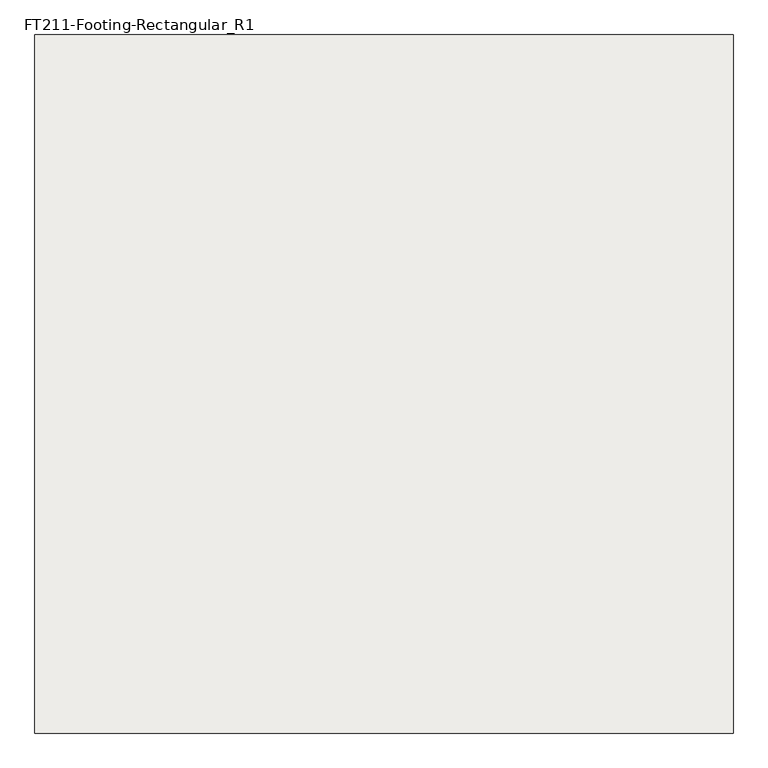
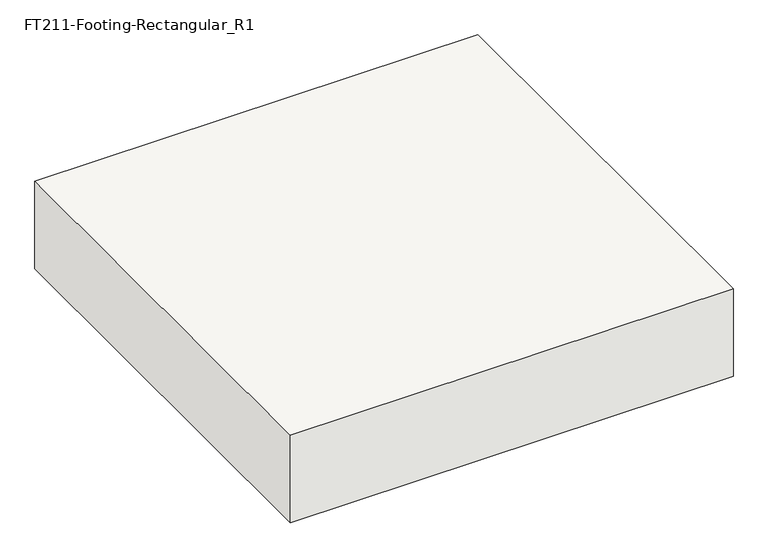
"""IFC4 building model written with IfcOpenShell, lengths in millimetres: slab geometry, FT211-Footing-Rectangular_R1 : H_SF_ACF_W2400xL2400xT500_Bitumen."""

import ifcopenshell
import ifcopenshell.guid

model = None  # the IFC model being written
_history = None  # IfcOwnerHistory: only IFC2X3 demands one
_inside = {}  # id of a spatial element -> (the spatial element, [elements in it])
_under = {}  # id of a project, library or spatial element -> (it, [spatial elements below it])
_declared = {}  # id of a project -> (the project, [libraries it declares])
_typed = {}  # id of a type object -> (the type object, [elements of that type])
_made_of = {}  # id of a material, layer set ... -> (it, [elements and type objects made of it])


def new_model(schema):
    """Start an empty IFC model of exactly this schema.

    Asked for "IFC4X3", IfcOpenShell would pick the latest addendum, in which some entities
    have other attributes; the version numbers below select the first issue.
    IFC2X3 requires an IfcOwnerHistory on every rooted entity: one is made here for all.
    """
    global model, _history
    if schema == "IFC4X3":
        model = ifcopenshell.file(schema_version=(4, 3, 0, 0))
    else:
        model = ifcopenshell.file(schema=schema)
    _inside.clear()
    _under.clear()
    _declared.clear()
    _typed.clear()
    _made_of.clear()
    _history = None
    if model.schema == "IFC2X3":
        org = make("IfcOrganization", Name="unknown")
        user = make(
            "IfcPersonAndOrganization",
            ThePerson=make("IfcPerson", FamilyName="unknown"),
            TheOrganization=org,
        )
        app = make(
            "IfcApplication",
            ApplicationDeveloper=org,
            Version="unknown",
            ApplicationFullName="unknown",
            ApplicationIdentifier="unknown",
        )
        _history = make(
            "IfcOwnerHistory",
            OwningUser=user,
            OwningApplication=app,
            ChangeAction="ADDED",
            CreationDate=0,
        )
    return model


def make(cls, **values):
    """One entity of the class cls with the attributes given. An attribute that is None is left unset."""
    return model.create_entity(
        cls, **{name: value for name, value in values.items() if value is not None}
    )


def rooted(cls, **values):
    """An entity with a GlobalId (a new one), such as an element, a storey or a relation."""
    return make(cls, GlobalId=ifcopenshell.guid.new(), OwnerHistory=_history, **values)


def si_unit(unit_type, name, prefix=None):
    """IfcSIUnit, for example si_unit("LENGTHUNIT", "METRE", prefix="MILLI")."""
    return make("IfcSIUnit", UnitType=unit_type, Prefix=prefix, Name=name)


def assignment(units):
    """IfcUnitAssignment: the units of a project."""
    return None if units is None else make("IfcUnitAssignment", Units=units)


def point(xyz):
    """IfcCartesianPoint."""
    return None if xyz is None else make("IfcCartesianPoint", Coordinates=xyz)


def direction(xyz):
    """IfcDirection."""
    return None if xyz is None else make("IfcDirection", DirectionRatios=xyz)


def frame(location, z_axis=None, x_axis=None):
    """IfcAxis2Placement3D, a coordinate frame: its origin and axes. An axis left out is left unset."""
    return make(
        "IfcAxis2Placement3D",
        Location=point(location),
        Axis=direction(z_axis),
        RefDirection=direction(x_axis),
    )


def origin():
    """The frame at (0, 0, 0) with its axes left unset."""
    return frame((0.0, 0.0, 0.0))


def place(relative_to, where):
    """IfcLocalPlacement: puts the frame where relative to a parent placement (None: the world)."""
    return make(
        "IfcLocalPlacement", PlacementRelTo=relative_to, RelativePlacement=where
    )


def context(
    kind, dimensions, precision=None, world=None, true_north=None, identifier=None
):
    """IfcGeometricRepresentationContext, for example the 3D "Model" context."""
    return make(
        "IfcGeometricRepresentationContext",
        ContextIdentifier=identifier,
        ContextType=kind,
        CoordinateSpaceDimension=dimensions,
        Precision=precision,
        WorldCoordinateSystem=world,
        TrueNorth=true_north,
    )


def project(units=None, contexts=None):
    """IfcProject with its units and contexts."""
    return rooted(
        "IfcProject",
        Name="project",
        RepresentationContexts=contexts,
        UnitsInContext=assignment(units),
    )


def spatial(cls, under=None, at=None, **own):
    """A site, building, storey or space (cls), placed at a placement, below another one or the project."""
    s = rooted(cls, ObjectPlacement=at, **own)
    if under is not None:
        _under.setdefault(under.id(), (under, []))[1].append(s)
    return s


def polyline(points):
    """IfcPolyline through the points."""
    return make("IfcPolyline", Points=[point(p) for p in points])


def outline(outer, holes=None, kind="AREA"):
    """IfcArbitraryClosedProfileDef: a profile drawn as a closed curve; with holes, ...WithVoids."""
    if holes is None:
        return make("IfcArbitraryClosedProfileDef", ProfileType=kind, OuterCurve=outer)
    return make(
        "IfcArbitraryProfileDefWithVoids",
        ProfileType=kind,
        OuterCurve=outer,
        InnerCurves=holes,
    )


def extrude(swept, where, along, depth):
    """IfcExtrudedAreaSolid: the profile swept, set in the frame where, extruded along a direction by depth."""
    return make(
        "IfcExtrudedAreaSolid",
        SweptArea=swept,
        Position=where,
        ExtrudedDirection=direction(along),
        Depth=depth,
    )


def shape(context_of_items, identifier, shape_type, items):
    """IfcShapeRepresentation: the items that make up one representation, for example the "Body"."""
    return make(
        "IfcShapeRepresentation",
        ContextOfItems=context_of_items,
        RepresentationIdentifier=identifier,
        RepresentationType=shape_type,
        Items=items,
    )


def source(mapping_origin, context_of_items, identifier, shape_type, items):
    """IfcRepresentationMap: a shape defined once, which mapped items show again and again."""
    return make(
        "IfcRepresentationMap",
        MappingOrigin=mapping_origin,
        MappedRepresentation=shape(context_of_items, identifier, shape_type, items),
    )


def transform(
    local_origin,
    x_axis=None,
    y_axis=None,
    z_axis=None,
    scale=None,
    scale2=None,
    scale3=None,
    uniform=True,
):
    """IfcCartesianTransformationOperator3D, or its non-uniform kind. x_axis, y_axis, z_axis: its Axis1, 2, 3."""
    if uniform:
        return make(
            "IfcCartesianTransformationOperator3D",
            Axis1=direction(x_axis),
            Axis2=direction(y_axis),
            LocalOrigin=point(local_origin),
            Scale=scale,
            Axis3=direction(z_axis),
        )
    return make(
        "IfcCartesianTransformationOperator3DnonUniform",
        Axis1=direction(x_axis),
        Axis2=direction(y_axis),
        LocalOrigin=point(local_origin),
        Scale=scale,
        Axis3=direction(z_axis),
        Scale2=scale2,
        Scale3=scale3,
    )


def mapped(mapping_source, mapping_target):
    """IfcMappedItem: shows the shape of a source again, moved by a transform."""
    return make(
        "IfcMappedItem", MappingSource=mapping_source, MappingTarget=mapping_target
    )


def made_of(thing, what):
    """Note that an element or type object is made of a material, layer set ...; save() writes the relation."""
    if what is not None:
        _made_of.setdefault(what.id(), (what, []))[1].append(thing)
    return thing


def element(
    cls,
    number,
    at=None,
    inside=None,
    cuts=None,
    type_object=None,
    material=None,
    context=None,
    identifier="Body",
    shape_type=None,
    held_by="IfcProductDefinitionShape",
    body=None,
    shapes=None,
    **own,
):
    """One element of the class cls, such as IfcWall. Its Tag is "e" and its number.

    at: its placement. inside: the storey or other place that contains it. cuts: it is an
    opening in that element (IfcRelVoidsElement). A single representation is given by context,
    identifier, shape_type and body (its items); several are given by shapes. held_by: the class
    of the entity that holds the representations. save() writes the other relations.
    """
    e = rooted(cls, Tag="e%d" % number, ObjectPlacement=at, **own)
    if body is not None:
        shapes = [shape(context, identifier, shape_type, body)]
    if shapes is not None:
        e.Representation = make(held_by, Representations=shapes)
    if inside is not None:
        _inside.setdefault(inside.id(), (inside, []))[1].append(e)
    if cuts is not None:
        rooted(
            "IfcRelVoidsElement", RelatingBuildingElement=cuts, RelatedOpeningElement=e
        )
    if type_object is not None:
        _typed.setdefault(type_object.id(), (type_object, []))[1].append(e)
    return made_of(e, material)


def aggregate(whole, parts):
    """IfcRelAggregates: a whole, such as a stair, and the parts it consists of."""
    return rooted("IfcRelAggregates", RelatingObject=whole, RelatedObjects=parts)


def save(model, path):
    """Write the relations noted so far, then the file.

    IfcRelAggregates (storeys below a building ...), IfcRelContainedInSpatialStructure (elements
    in a storey), IfcRelDefinesByType, IfcRelAssociatesMaterial and IfcRelDeclares: one each for
    every whole, place, type object, material and project.
    """
    for whole, parts in _under.values():
        aggregate(whole, parts)
    for where, things in _inside.values():
        rooted(
            "IfcRelContainedInSpatialStructure",
            RelatedElements=things,
            RelatingStructure=where,
        )
    for kind, things in _typed.values():
        rooted("IfcRelDefinesByType", RelatedObjects=things, RelatingType=kind)
    for what, things in _made_of.values():
        rooted("IfcRelAssociatesMaterial", RelatedObjects=things, RelatingMaterial=what)
    for by, libraries in _declared.values():
        rooted("IfcRelDeclares", RelatingContext=by, RelatedDefinitions=libraries)
    model.write(path)


def ft211_footing_rectangular_r1_5fe39465(model_context):
    return source(origin(), model_context, "Body", "SweptSolid", [
        extrude(outline(polyline([(1200.0, 1200.0), (1200.0, -1200.0), (-1200.0, -1200.0), (-1200.0, 1200.0), (1200.0, 1200.0)])), frame((0.0, 0.0, -500.0), z_axis=(0.0, 0.0, 1.0), x_axis=(1.0, 0.0, 0.0)), (0.0, 0.0, 1.0), 500.0),
    ])


if __name__ == "__main__":
    model = new_model("IFC4")
    model_context = context("Model", 3, world=origin())
    ifc_project = project(units=[si_unit("LENGTHUNIT", "METRE", prefix="MILLI")], contexts=[model_context])
    site = spatial("IfcSite", under=ifc_project)
    building = spatial("IfcBuilding", under=site)
    placement = place(None, origin())
    ft211_footing_rectangular_r1_shape = ft211_footing_rectangular_r1_5fe39465(model_context)
    element("IfcSlab", 1, ObjectType="FT211-Footing-Rectangular_R1 : H_SF_ACF_W2400xL2400xT500_Bitumen", at=placement, inside=building, context=model_context, shape_type="MappedRepresentation", body=[
        mapped(ft211_footing_rectangular_r1_shape, transform((0.0, 0.0, 0.0), x_axis=(1.0, 0.0, 0.0), y_axis=(0.0, 1.0, 0.0), z_axis=(0.0, 0.0, 1.0))),
    ])
    save(model, "model.ifc")

# Revit data of these elements
# Type "FT211-Footing-Rectangular_R1 : H_SF_ACF_W2400xL2400xT500_Bitumen"
#   Top bar = "D25@300"
#   Description = "UG Shallow Foundation"
#   Bottom bar = "D20@300"
#   Width = 2400.000 mm
#   Length = 2400.000 mm
#   Foundation Thickness = 500.000 mm
#   Structural Material [instance default] = none
#   Assembly Code = ""
